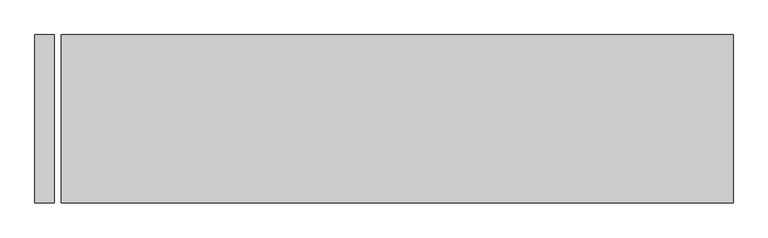
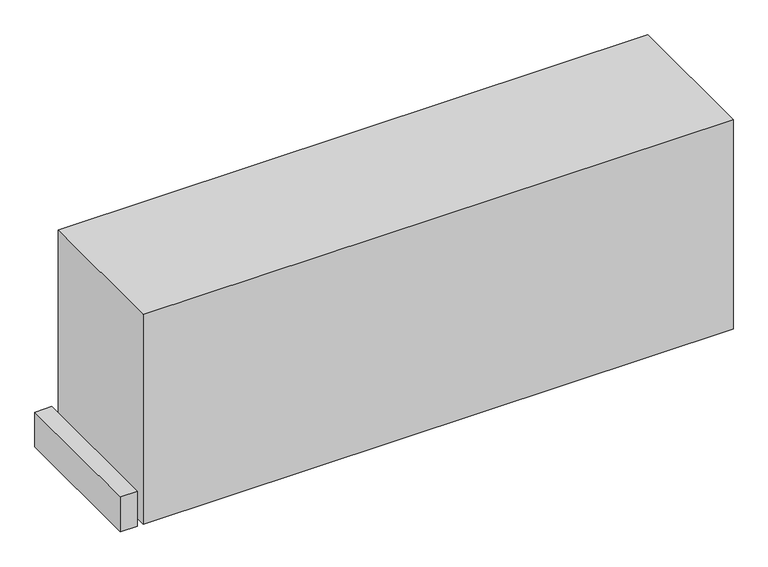
"""IFC4 building model written with IfcOpenShell, lengths in millimetres: proxy geometry, Generic Models 291:Generic Models 291:154945 : Generic Models 291:Generic Models 291:154945."""

from ifc_helpers import new_model, si_unit, origin, origin_with_axes, place, context, project, spatial, polyline, outline, extrude, source, transform, mapped, element, save


def generic_models_807a6788(model_context):
    return source(origin(), model_context, "Body", "SweptSolid", [
        extrude(outline(polyline([(8351.0918069, 8709.7928291), (8351.0918069, 8404.9928291), (7134.103213, 8404.9928291), (7134.103213, 8709.7928291), (8351.0918069, 8709.7928291)])), origin_with_axes(), (0.0, 0.0, 1.0), 457.2),
        extrude(outline(polyline([(7121.403213, 8709.7928291), (7121.403213, 8404.9928291), (7086.3961993, 8404.9928291), (7086.3961993, 8709.7928291), (7121.403213, 8709.7928291)])), origin_with_axes(), (0.0, 0.0, 1.0), 76.2),
    ])


if __name__ == "__main__":
    model = new_model("IFC4")
    model_context = context("Model", 3, world=origin())
    ifc_project = project(units=[si_unit("LENGTHUNIT", "METRE", prefix="MILLI")], contexts=[model_context])
    site = spatial("IfcSite", under=ifc_project)
    building = spatial("IfcBuilding", under=site)
    placement = place(None, origin())
    generic_models_shape = generic_models_807a6788(model_context)
    element("IfcBuildingElementProxy", 1, Name="Generic Models 291:Generic Models 291:154945 : Generic Models 291:Generic Models 291:154945", ObjectType="Generic Models 291:Generic Models 291:154945 : Generic Models 291:Generic Models 291:154945", at=placement, inside=building, context=model_context, shape_type="MappedRepresentation", body=[
        mapped(generic_models_shape, transform((0.0, 0.0, 0.0), x_axis=(1.0, 0.0, 0.0), y_axis=(0.0, 1.0, 0.0), z_axis=(0.0, 0.0, 1.0))),
    ])
    save(model, "model.ifc")

# Revit data of these elements
# Type "Generic Models 291:Generic Models 291:154945 : Generic Models 291:Generic Models 291:154945"
#   NameOverride = "Generic Models 291:Generic Models 291:154945"
#   ObjectTypeOverride = "Generic Models 291:Generic Models 291"
#   Reference = "Generic Models 291"
#   Category = "Generic Models"
#   Tag = "154945"
# Element 1 (IfcBuildingElementProxy, "Generic Models 291:Generic Models 291:154945 : Generic Models 291:Generic Models 291:154945")
#   Materials on its faces: "_CONCRETE SLAB W/ WIRE MESH (SEE STRUCT. DWGS) - SLOPE 1% AWAY FROM BUILDING 9884"
# Materials
#   "_CONCRETE SLAB W/ WIRE MESH (SEE STRUCT. DWGS) - SLOPE 1% AWAY FROM BUILDING 9884": class "Unassigned", colour RGB 191 191 191, transparency 0
